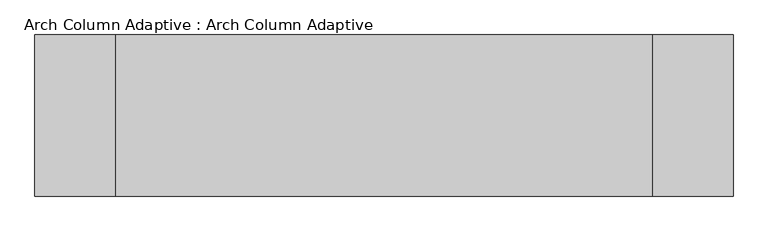
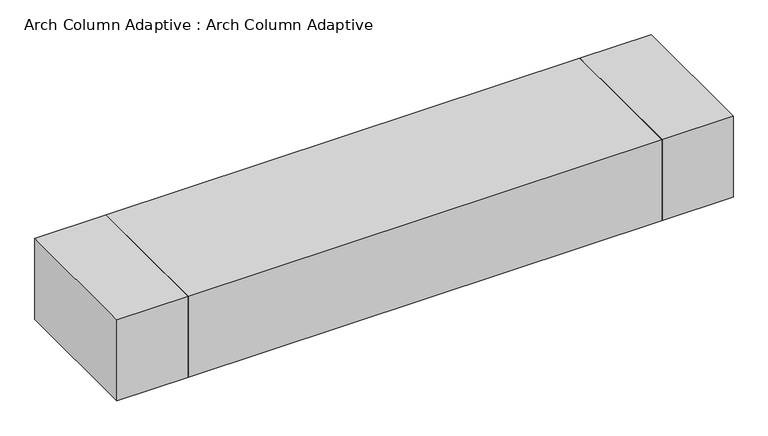
"""IFC4 building model written with IfcOpenShell, lengths in millimetres: proxy geometry, Arch Column Adaptive : Arch Column Adaptive."""

from ifc_helpers import new_model, si_unit, frame, origin, place, context, project, spatial, polyline, outline, extrude, source, transform, mapped, element, save


def arch_column_adaptive_arch_column_adaptive_84170001(model_context):
    return source(origin(), model_context, "Body", "SweptSolid", [
        extrude(outline(polyline([(5000.0, -1500.0), (5000.0, 1500.0), (6500.0, 1500.0), (6500.0, -1500.0), (5000.0, -1500.0)])), frame((0.0, 0.0, 8880.0), z_axis=(0.0, 0.0, 1.0), x_axis=(1.0, 0.0, 0.0)), (0.0, 0.0, 1.0), 1800.0),
        extrude(outline(polyline([(-5000.0, 1500.0), (-5000.0, -1500.0), (-6500.0, -1500.0), (-6500.0, 1500.0), (-5000.0, 1500.0)])), frame((0.0, 0.0, 8880.0), z_axis=(0.0, 0.0, 1.0), x_axis=(1.0, 0.0, 0.0)), (0.0, 0.0, 1.0), 1800.0),
        extrude(outline(polyline([(-5000.0, -1500.0), (-5000.0, 1500.0), (5000.0, 1500.0), (5000.0, -1500.0), (-5000.0, -1500.0)])), frame((0.0, 0.0, 8880.0), z_axis=(0.0, 0.0, 1.0), x_axis=(1.0, 0.0, 0.0)), (0.0, 0.0, 1.0), 1800.0),
    ])


if __name__ == "__main__":
    model = new_model("IFC4")
    model_context = context("Model", 3, world=origin())
    ifc_project = project(units=[si_unit("LENGTHUNIT", "METRE", prefix="MILLI")], contexts=[model_context])
    site = spatial("IfcSite", under=ifc_project)
    building = spatial("IfcBuilding", under=site)
    placement = place(None, origin())
    arch_column_adaptive_arch_column_adaptive_shape = arch_column_adaptive_arch_column_adaptive_84170001(model_context)
    element("IfcBuildingElementProxy", 1, Name="Arch Column Adaptive : Arch Column Adaptive", ObjectType="Arch Column Adaptive : Arch Column Adaptive", at=placement, inside=building, context=model_context, shape_type="MappedRepresentation", body=[
        mapped(arch_column_adaptive_arch_column_adaptive_shape, transform((0.0, 0.0, 0.0), x_axis=(1.0, 0.0, 0.0), y_axis=(0.0, 1.0, 0.0), z_axis=(0.0, 0.0, 1.0))),
    ])
    save(model, "model.ifc")

# Revit data of these elements
# Type "Arch Column Adaptive : Arch Column Adaptive"
#   Top Width = 3000 mm
#   Length [instance default] = 21000 mm
#   Height [instance default] = 50000 mm
#   Default Elevation = 0
# Element 1 (IfcBuildingElementProxy, "Arch Column Adaptive : Arch Column Adaptive")
#   Height = 8880 mm
